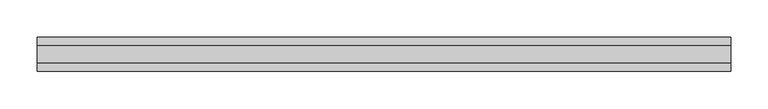
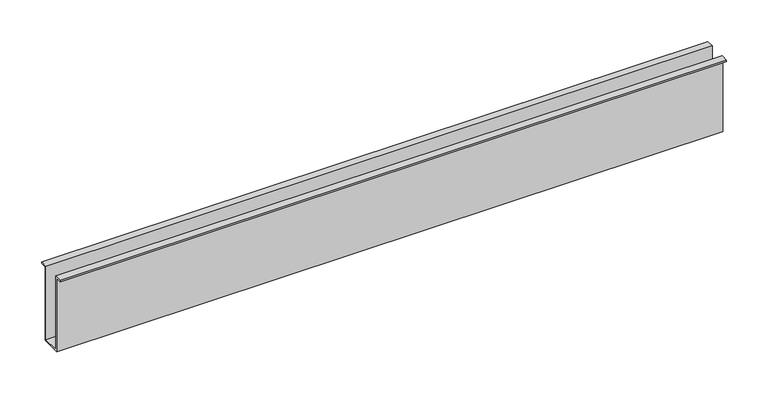
"""IFC4 building model written with IfcOpenShell, lengths in millimetres: railing geometry, ML_Perfil U de embutir4 : ML_Perfil U de embutir."""

import ifcopenshell
import ifcopenshell.guid

model = None  # the IFC model being written
_history = None  # IfcOwnerHistory: only IFC2X3 demands one
_inside = {}  # id of a spatial element -> (the spatial element, [elements in it])
_under = {}  # id of a project, library or spatial element -> (it, [spatial elements below it])
_declared = {}  # id of a project -> (the project, [libraries it declares])
_typed = {}  # id of a type object -> (the type object, [elements of that type])
_made_of = {}  # id of a material, layer set ... -> (it, [elements and type objects made of it])


def new_model(schema):
    """Start an empty IFC model of exactly this schema.

    Asked for "IFC4X3", IfcOpenShell would pick the latest addendum, in which some entities
    have other attributes; the version numbers below select the first issue.
    IFC2X3 requires an IfcOwnerHistory on every rooted entity: one is made here for all.
    """
    global model, _history
    if schema == "IFC4X3":
        model = ifcopenshell.file(schema_version=(4, 3, 0, 0))
    else:
        model = ifcopenshell.file(schema=schema)
    _inside.clear()
    _under.clear()
    _declared.clear()
    _typed.clear()
    _made_of.clear()
    _history = None
    if model.schema == "IFC2X3":
        org = make("IfcOrganization", Name="unknown")
        user = make(
            "IfcPersonAndOrganization",
            ThePerson=make("IfcPerson", FamilyName="unknown"),
            TheOrganization=org,
        )
        app = make(
            "IfcApplication",
            ApplicationDeveloper=org,
            Version="unknown",
            ApplicationFullName="unknown",
            ApplicationIdentifier="unknown",
        )
        _history = make(
            "IfcOwnerHistory",
            OwningUser=user,
            OwningApplication=app,
            ChangeAction="ADDED",
            CreationDate=0,
        )
    return model


def make(cls, **values):
    """One entity of the class cls with the attributes given. An attribute that is None is left unset."""
    return model.create_entity(
        cls, **{name: value for name, value in values.items() if value is not None}
    )


def rooted(cls, **values):
    """An entity with a GlobalId (a new one), such as an element, a storey or a relation."""
    return make(cls, GlobalId=ifcopenshell.guid.new(), OwnerHistory=_history, **values)


def si_unit(unit_type, name, prefix=None):
    """IfcSIUnit, for example si_unit("LENGTHUNIT", "METRE", prefix="MILLI")."""
    return make("IfcSIUnit", UnitType=unit_type, Prefix=prefix, Name=name)


def assignment(units):
    """IfcUnitAssignment: the units of a project."""
    return None if units is None else make("IfcUnitAssignment", Units=units)


def point(xyz):
    """IfcCartesianPoint."""
    return None if xyz is None else make("IfcCartesianPoint", Coordinates=xyz)


def direction(xyz):
    """IfcDirection."""
    return None if xyz is None else make("IfcDirection", DirectionRatios=xyz)


def frame(location, z_axis=None, x_axis=None):
    """IfcAxis2Placement3D, a coordinate frame: its origin and axes. An axis left out is left unset."""
    return make(
        "IfcAxis2Placement3D",
        Location=point(location),
        Axis=direction(z_axis),
        RefDirection=direction(x_axis),
    )


def origin():
    """The frame at (0, 0, 0) with its axes left unset."""
    return frame((0.0, 0.0, 0.0))


def place(relative_to, where):
    """IfcLocalPlacement: puts the frame where relative to a parent placement (None: the world)."""
    return make(
        "IfcLocalPlacement", PlacementRelTo=relative_to, RelativePlacement=where
    )


def context(
    kind, dimensions, precision=None, world=None, true_north=None, identifier=None
):
    """IfcGeometricRepresentationContext, for example the 3D "Model" context."""
    return make(
        "IfcGeometricRepresentationContext",
        ContextIdentifier=identifier,
        ContextType=kind,
        CoordinateSpaceDimension=dimensions,
        Precision=precision,
        WorldCoordinateSystem=world,
        TrueNorth=true_north,
    )


def project(units=None, contexts=None):
    """IfcProject with its units and contexts."""
    return rooted(
        "IfcProject",
        Name="project",
        RepresentationContexts=contexts,
        UnitsInContext=assignment(units),
    )


def spatial(cls, under=None, at=None, **own):
    """A site, building, storey or space (cls), placed at a placement, below another one or the project."""
    s = rooted(cls, ObjectPlacement=at, **own)
    if under is not None:
        _under.setdefault(under.id(), (under, []))[1].append(s)
    return s


def polyline(points):
    """IfcPolyline through the points."""
    return make("IfcPolyline", Points=[point(p) for p in points])


def outline(outer, holes=None, kind="AREA"):
    """IfcArbitraryClosedProfileDef: a profile drawn as a closed curve; with holes, ...WithVoids."""
    if holes is None:
        return make("IfcArbitraryClosedProfileDef", ProfileType=kind, OuterCurve=outer)
    return make(
        "IfcArbitraryProfileDefWithVoids",
        ProfileType=kind,
        OuterCurve=outer,
        InnerCurves=holes,
    )


def extrude(swept, where, along, depth):
    """IfcExtrudedAreaSolid: the profile swept, set in the frame where, extruded along a direction by depth."""
    return make(
        "IfcExtrudedAreaSolid",
        SweptArea=swept,
        Position=where,
        ExtrudedDirection=direction(along),
        Depth=depth,
    )


def shape(context_of_items, identifier, shape_type, items):
    """IfcShapeRepresentation: the items that make up one representation, for example the "Body"."""
    return make(
        "IfcShapeRepresentation",
        ContextOfItems=context_of_items,
        RepresentationIdentifier=identifier,
        RepresentationType=shape_type,
        Items=items,
    )


def source(mapping_origin, context_of_items, identifier, shape_type, items):
    """IfcRepresentationMap: a shape defined once, which mapped items show again and again."""
    return make(
        "IfcRepresentationMap",
        MappingOrigin=mapping_origin,
        MappedRepresentation=shape(context_of_items, identifier, shape_type, items),
    )


def transform(
    local_origin,
    x_axis=None,
    y_axis=None,
    z_axis=None,
    scale=None,
    scale2=None,
    scale3=None,
    uniform=True,
):
    """IfcCartesianTransformationOperator3D, or its non-uniform kind. x_axis, y_axis, z_axis: its Axis1, 2, 3."""
    if uniform:
        return make(
            "IfcCartesianTransformationOperator3D",
            Axis1=direction(x_axis),
            Axis2=direction(y_axis),
            LocalOrigin=point(local_origin),
            Scale=scale,
            Axis3=direction(z_axis),
        )
    return make(
        "IfcCartesianTransformationOperator3DnonUniform",
        Axis1=direction(x_axis),
        Axis2=direction(y_axis),
        LocalOrigin=point(local_origin),
        Scale=scale,
        Axis3=direction(z_axis),
        Scale2=scale2,
        Scale3=scale3,
    )


def mapped(mapping_source, mapping_target):
    """IfcMappedItem: shows the shape of a source again, moved by a transform."""
    return make(
        "IfcMappedItem", MappingSource=mapping_source, MappingTarget=mapping_target
    )


def made_of(thing, what):
    """Note that an element or type object is made of a material, layer set ...; save() writes the relation."""
    if what is not None:
        _made_of.setdefault(what.id(), (what, []))[1].append(thing)
    return thing


def element(
    cls,
    number,
    at=None,
    inside=None,
    cuts=None,
    type_object=None,
    material=None,
    context=None,
    identifier="Body",
    shape_type=None,
    held_by="IfcProductDefinitionShape",
    body=None,
    shapes=None,
    **own,
):
    """One element of the class cls, such as IfcWall. Its Tag is "e" and its number.

    at: its placement. inside: the storey or other place that contains it. cuts: it is an
    opening in that element (IfcRelVoidsElement). A single representation is given by context,
    identifier, shape_type and body (its items); several are given by shapes. held_by: the class
    of the entity that holds the representations. save() writes the other relations.
    """
    e = rooted(cls, Tag="e%d" % number, ObjectPlacement=at, **own)
    if body is not None:
        shapes = [shape(context, identifier, shape_type, body)]
    if shapes is not None:
        e.Representation = make(held_by, Representations=shapes)
    if inside is not None:
        _inside.setdefault(inside.id(), (inside, []))[1].append(e)
    if cuts is not None:
        rooted(
            "IfcRelVoidsElement", RelatingBuildingElement=cuts, RelatedOpeningElement=e
        )
    if type_object is not None:
        _typed.setdefault(type_object.id(), (type_object, []))[1].append(e)
    return made_of(e, material)


def aggregate(whole, parts):
    """IfcRelAggregates: a whole, such as a stair, and the parts it consists of."""
    return rooted("IfcRelAggregates", RelatingObject=whole, RelatedObjects=parts)


def save(model, path):
    """Write the relations noted so far, then the file.

    IfcRelAggregates (storeys below a building ...), IfcRelContainedInSpatialStructure (elements
    in a storey), IfcRelDefinesByType, IfcRelAssociatesMaterial and IfcRelDeclares: one each for
    every whole, place, type object, material and project.
    """
    for whole, parts in _under.values():
        aggregate(whole, parts)
    for where, things in _inside.values():
        rooted(
            "IfcRelContainedInSpatialStructure",
            RelatedElements=things,
            RelatingStructure=where,
        )
    for kind, things in _typed.values():
        rooted("IfcRelDefinesByType", RelatedObjects=things, RelatingType=kind)
    for what, things in _made_of.values():
        rooted("IfcRelAssociatesMaterial", RelatedObjects=things, RelatingMaterial=what)
    for by, libraries in _declared.values():
        rooted("IfcRelDeclares", RelatingContext=by, RelatedDefinitions=libraries)
    model.write(path)


def railing_24874f95(model_context):
    return source(origin(), model_context, "Body", "SweptSolid", [
        extrude(outline(polyline([(1832.4523952, 3702.0), (1832.4523952, 3594.0), (1856.4523952, 3594.0), (1856.4523952, 3702.0), (1866.9523952, 3702.0), (1866.9523952, 3700.0), (1858.4523952, 3700.0), (1858.4523952, 3592.0), (1830.4523952, 3592.0), (1830.4523952, 3700.0), (1821.9523952, 3700.0), (1821.9523952, 3702.0), (1832.4523952, 3702.0)])), frame((-12226.1487231, 0.0, 0.0), z_axis=(1.0, 0.0, 0.0), x_axis=(0.0, 1.0, 0.0)), (0.0, 0.0, 1.0), 925.0),
    ])


if __name__ == "__main__":
    model = new_model("IFC4")
    model_context = context("Model", 3, world=origin())
    ifc_project = project(units=[si_unit("LENGTHUNIT", "METRE", prefix="MILLI")], contexts=[model_context])
    site = spatial("IfcSite", under=ifc_project)
    building = spatial("IfcBuilding", under=site)
    placement = place(None, origin())
    railing_shape = railing_24874f95(model_context)
    element("IfcRailing", 1, ObjectType="ML_Perfil U de embutir4 : ML_Perfil U de embutir", at=placement, inside=building, context=model_context, shape_type="MappedRepresentation", body=[
        mapped(railing_shape, transform((0.0, 0.0, 0.0), x_axis=(1.0, 0.0, 0.0), y_axis=(0.0, 1.0, 0.0), z_axis=(0.0, 0.0, 1.0))),
    ])
    save(model, "model.ifc")

# Revit data of these elements
# Type "ML_Perfil U de embutir4 : ML_Perfil U de embutir"
#   ME_Compr [instance default] = 0.925 m
#   ME_Material Perfil [instance default] = .ALUMÍNIO COM PINTURA ELETROSTÁTICA BRANCA
# Element 1 (IfcRailing, "ML_Perfil U de embutir4 : ML_Perfil U de embutir")
#   Materials on its faces: ".ALUMÍNIO COM PINTURA ELETROSTÁTICA BRANCA"
# Materials
#   ".ALUMÍNIO COM PINTURA ELETROSTÁTICA BRANCA": class "CC_METAIS", colour RGB 241 241 241, transparency 0, Cost = 0
